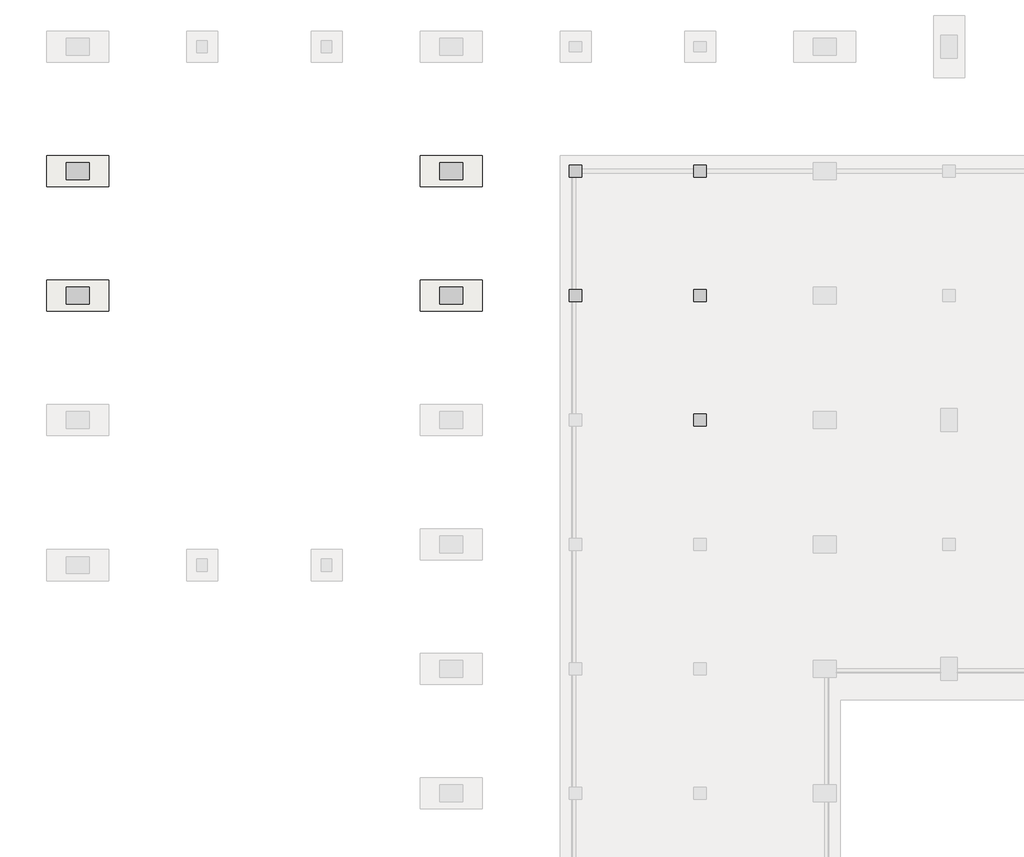
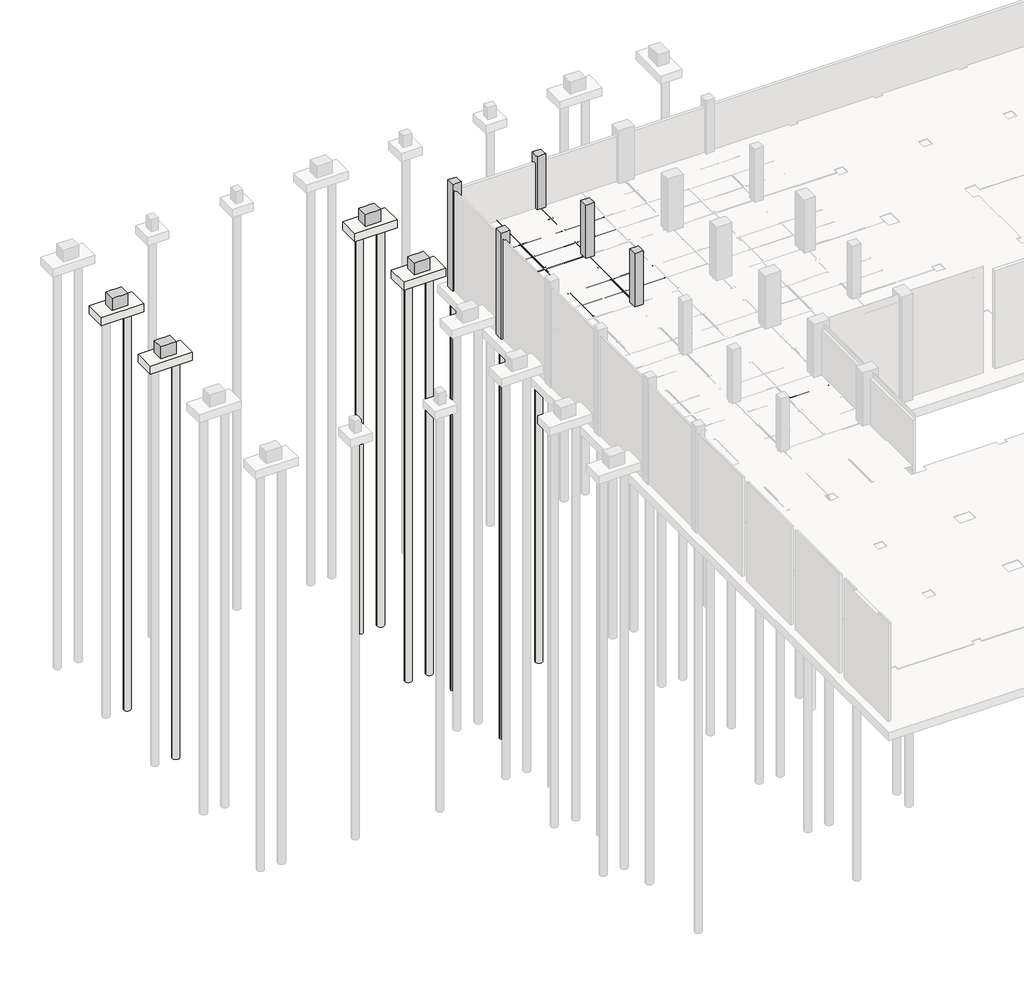
# Not in any storey, part 8 of 16: 24 beams, 13 slabs, 9 columns.
# Revit data of these elements (continued)
# Type "Steel Framing_H_KS : H_SB_AR_S02_H-400x200x8x13_BSG1" (continued)
#   Perimeter = 1.56 m²/m
#   Nominal Weight = 66.00 kgf/m
#   Moment of Inertia weak axis = 1740.00 cm⁴
#   Moment of Inertia strong axis = 23700.00 cm⁴
#   Height = 40.0 cm
#   Flange Thickness = 1.3 cm
#   Elastic Modulus weak axis = 174.0 cm³
#   Elastic Modulus strong axis = 1190.0 cm³
#   Centroid Vertical = 20.0 cm
#   Centroid Horizontal = 10.0 cm
#   Bolt Spacing = 8.89 cm
#   Length [instance default] = 1500 mm
#   Structural Material [instance default] = Steel, 45-345
#   Section Name Key = ""
#   Assembly Code = ""
# Type "Steel Framing_H_KS : H_SB_AR_S02_H-400x200x8x13_BSG2"
#   Type Comments = "MAIN"
#   Type Mark = "BSG2"
#   H_SectionID = "H-400x200x8x13"
#   H_Ratio for Additional Steel Plate = 0.2
#   Width = 20.0 cm
#   Web Thickness = 0.8 cm
#   Web Fillet = 1.6 cm
#   Warping Constant = 649000.0 cm⁶
#   Torsional Moment of Inertia = 35.8981 cm⁴
#   Section Area = 84.12 cm²
#   Plastic Modulus weak axis = 268.0 cm³
#   Plastic Modulus strong axis = 1330.0 cm³
#   Perimeter = 1.56 m²/m
#   Nominal Weight = 66.00 kgf/m
#   Moment of Inertia weak axis = 1740.00 cm⁴
#   Moment of Inertia strong axis = 23700.00 cm⁴
#   Height = 40.0 cm
#   Flange Thickness = 1.3 cm
#   Elastic Modulus weak axis = 174.0 cm³
#   Elastic Modulus strong axis = 1190.0 cm³
#   Centroid Vertical = 20.0 cm
#   Centroid Horizontal = 10.0 cm
#   Bolt Spacing = 8.89 cm
#   Length [instance default] = 1500 mm
#   Structural Material [instance default] = Steel, 45-345
#   Section Name Key = ""
#   Assembly Code = ""
# Type "Steel Framing_H_KS : H_SB_AR_S02_H-400x200x8x13_BSB1"
#   Type Comments = "MAIN"
#   Type Mark = "BSB1"
#   H_SectionID = "H-400x200x8x13"
#   H_Ratio for Additional Steel Plate = 0.2
#   Width = 20.0 cm
#   Web Thickness = 0.8 cm
#   Web Fillet = 1.6 cm
#   Warping Constant = 649000.0 cm⁶
#   Torsional Moment of Inertia = 35.8981 cm⁴
#   Section Area = 84.12 cm²
#   Plastic Modulus weak axis = 268.0 cm³
#   Plastic Modulus strong axis = 1330.0 cm³
#   Perimeter = 1.56 m²/m
#   Nominal Weight = 66.00 kgf/m
#   Moment of Inertia weak axis = 1740.00 cm⁴
#   Moment of Inertia strong axis = 23700.00 cm⁴
#   Height = 40.0 cm
#   Flange Thickness = 1.3 cm
#   Elastic Modulus weak axis = 174.0 cm³
#   Elastic Modulus strong axis = 1190.0 cm³
#   Centroid Vertical = 20.0 cm
#   Centroid Horizontal = 10.0 cm
#   Bolt Spacing = 8.89 cm
#   Length [instance default] = 1500 mm
#   Structural Material [instance default] = Steel, 45-345
#   Section Name Key = ""
#   Assembly Code = ""
# Type "Steel Framing_C_KS : H_SB_AR_S02_C-150x75x6.5x10_J1"
#   Type Mark = "J1"
#   H_SectionID = "C-150x75x6.5x10"
#   Assembly Code = "B10"
#   H_Ratio for Additional Steel Plate = 0.2
#   Perimeter = 0.51 m²/m
#   Nominal Weight = 18.60 kgf/m
#   Length [instance default] = 1000 mm
#   bf = 75 mm
#   d = 150 mm
#   tf = 10 mm
#   tw = 6.5 mm
#   x = 22.8 mm
#   A = 0.002371 m²
#   Structural Material [instance default] = Steel, 45-345
# Type "RC_Column_Rectangular : H_SC_AR_S15_UG PED_Bit_800x1100_PD1"
#   Type Mark = "PD1"
#   Type Comments = "UG"
#   H_SectionID = "600 x 900"
#   H_Rebar Ratio = 0.3
#   Width = 800 mm
#   Depth = 1100 mm
#   hec_material3 [instance default] = none
#   hec_material2 [instance default] = none
#   hec_material1 [instance default] = none
#   Structural Material [instance default] = none
#   Description = (empty or 0)
# Type "RC_Column_Rectangular : H_SC_AR_S15_UG PED_Bit_600x600_BC1"
#   Type Mark = "BC1"
#   Type Comments = "UG"
#   H_SectionID = "600 x 600"
#   H_Rebar Ratio = 0.3
#   Width = 600 mm
#   Depth = 600 mm
#   hec_material3 [instance default] = none
#   hec_material2 [instance default] = none
#   hec_material1 [instance default] = none
#   Structural Material [instance default] = none
#   Description = (empty or 0)
# Type "Foundation Rectangular (Non-Pile) : H_SF_AR_S18_Shallow Fdn_Bitumen_1500x3000xT600_F1"
#   Type Comments = "UG"
#   Type Mark = "F1"
#   Top bar = "D25@300"
#   Description = "UG Shallow Foundation"
#   Bottom bar = "D20@300"
#   H_Rebar Ratio = 0.12
#   Width = 1500 mm
#   Length = 3000 mm
#   Foundation Thickness = 600 mm
#   Structural Material [instance default] = none
#   Assembly Code = ""
# Type "PILE : H_SF_AR_S19_PHC Pile_Pre-boring_D500_L30"
#   Assembly Code = "A1020120"
#   반지름 = 250 mm
#   최소 내포 = 150 mm
#   Diameter = 500 mm
#   Depth = 30000 mm
#   Structural Material [instance default] = none
# Element 1 (IfcBeam, "Steel Framing_H_KS : H_SB_AR_S02_H-400x200x8x13_BSG1")
#   Structural Material = Steel, 45-345
#   Phase Created = New Construction
#   Materials on its faces: "Steel, 45-345"
# Elements 2, 13 (IfcBeam, "Steel Framing_H_KS : H_SB_AR_S02_H-400x200x8x13_BSG2")
#   Structural Material = Steel, 45-345
#   Phase Created = New Construction
#   Materials on its faces: "Steel, 45-345"
# Elements 3, 14 (IfcBeam, "Steel Framing_H_KS : H_SB_AR_S02_H-400x200x8x13_BSB1")
#   Structural Material = Steel, 45-345
#   Phase Created = New Construction
#   Materials on its faces: "Steel, 45-345"
# Elements 4, 5, 6, 7, 8, 9, 10, 11, 12, 15, 16, 17, 18, 19, 20, 21, 22, 23, 24 (IfcBeam, "Steel Framing_C_KS : H_SB_AR_S02_C-150x75x6.5x10_J1")
#   Structural Material = Steel, 45-345
#   Phase Created = New Construction
#   Materials on its faces: "Steel, 45-345"
# Elements 25, 26, 27, 28 (IfcColumn, "RC_Column_Rectangular : H_SC_AR_S15_UG PED_Bit_800x1100_PD1")
#   Comments = ""
#   hec_material3 = none
#   hec_material2 = none
#   hec_material1 = none
#   Structural Material = 00_Concrete_Reinf. Conc.
#   Phase Created = New Construction
#   Materials on its faces: "00_Concrete_Reinf. Conc."
# Elements 29, 30, 31, 32, 33 (IfcColumn, "RC_Column_Rectangular : H_SC_AR_S15_UG PED_Bit_600x600_BC1")
#   Comments = ""
#   hec_material3 = none
#   hec_material2 = none
#   hec_material1 = none
#   Structural Material = 00_Concrete_Reinf. Conc.
#   Phase Created = New Construction
#   Materials on its faces: "00_Concrete_Reinf. Conc."
# Elements 34, 35, 36, 37 (IfcSlab, "Foundation Rectangular (Non-Pile) : H_SF_AR_S18_Shallow Fdn_Bitumen_1500x3000xT600_F1")
#   Comments = ""
#   Structural Material = 00_Concrete_Reinf. Conc.
#   Phase Created = New Construction
#   Materials on its faces: "00_Concrete_Reinf. Conc."
# Elements 38, 39, 40, 41, 42, 43 (IfcSlab, "PILE : H_SF_AR_S19_PHC Pile_Pre-boring_D500_L30")
#   Structural Material = Concrete, Precast
#   Phase Created = New Construction
#   Materials on its faces: "Concrete, Precast"
# Elements 44, 45, 46 (IfcSlab, "PILE : H_SF_AR_S19_PHC Pile_Pre-boring_D500_L30")
#   Structural Material = none
#   Phase Created = New Construction
# Materials
#   "Steel, 45-345": class "Metal", colour RGB 189 187 185, transparency 0, Description = "Steel 345 MPa", Cost = 0
#   "00_Concrete_Reinf. Conc.": class "Concrete", colour RGB 176 176 176, transparency 0, Description = "Reinf. Conc.", Cost = 0, Image = Concrete.Cast-In-Place.Flat.Polished.Grey.jpg
#   "Concrete, Precast": class "Concrete", colour RGB 115 116 108, transparency 0, Description = "Precast concrete", Cost = 0
